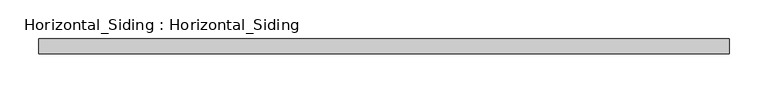
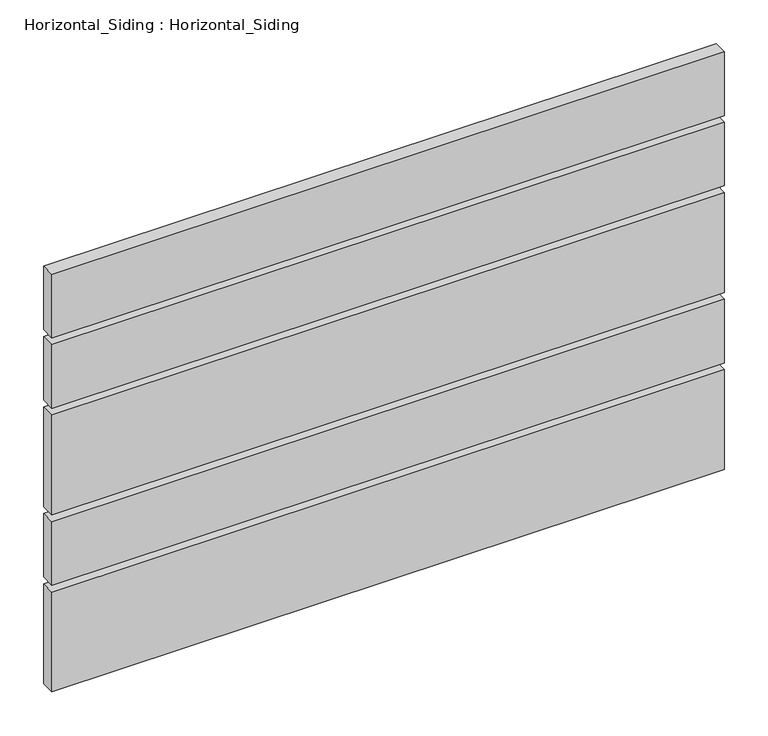
"""IFC4 building model written with IfcOpenShell, lengths in millimetres: plate geometry, Horizontal_Siding : Horizontal_Siding."""

from ifc_helpers import new_model, si_unit, frame, origin, place, context, project, spatial, polyline, outline, extrude, source, transform, mapped, element, save


def horizontal_siding_horizontal_siding_71e25863(model_context):
    return source(origin(), model_context, "Body", "SweptSolid", [
        extrude(outline(polyline([(444.5598994, -19.05), (-444.5598994, -19.05), (-444.5598994, 0.0), (444.5598994, 0.0), (444.5598994, -19.05)])), frame((0.0, 0.0, 9.525), z_axis=(0.0, 0.0, 1.0), x_axis=(1.0, 0.0, 0.0)), (0.0, 0.0, 1.0), 139.7),
        extrude(outline(polyline([(444.5598994, -19.05), (-444.5598994, -19.05), (-444.5598994, 0.0), (444.5598994, 0.0), (444.5598994, -19.05)])), frame((0.0, 0.0, 158.75), z_axis=(0.0, 0.0, 1.0), x_axis=(1.0, 0.0, 0.0)), (0.0, 0.0, 1.0), 88.9),
        extrude(outline(polyline([(444.5598994, -19.05), (-444.5598994, -19.05), (-444.5598994, 0.0), (444.5598994, 0.0), (444.5598994, -19.05)])), frame((0.0, 0.0, 257.175), z_axis=(0.0, 0.0, 1.0), x_axis=(1.0, 0.0, 0.0)), (0.0, 0.0, 1.0), 139.7),
        extrude(outline(polyline([(444.5598994, -19.05), (-444.5598994, -19.05), (-444.5598994, 0.0), (444.5598994, 0.0), (444.5598994, -19.05)])), frame((0.0, 0.0, 406.4), z_axis=(0.0, 0.0, 1.0), x_axis=(1.0, 0.0, 0.0)), (0.0, 0.0, 1.0), 88.9),
        extrude(outline(polyline([(444.5598994, -19.05), (-444.5598994, -19.05), (-444.5598994, 0.0), (444.5598994, 0.0), (444.5598994, -19.05)])), frame((0.0, 0.0, 504.825), z_axis=(0.0, 0.0, 1.0), x_axis=(1.0, 0.0, 0.0)), (0.0, 0.0, 1.0), 88.9),
    ])


if __name__ == "__main__":
    model = new_model("IFC4")
    model_context = context("Model", 3, world=origin())
    ifc_project = project(units=[si_unit("LENGTHUNIT", "METRE", prefix="MILLI")], contexts=[model_context])
    site = spatial("IfcSite", under=ifc_project)
    building = spatial("IfcBuilding", under=site)
    placement = place(None, origin())
    horizontal_siding_horizontal_siding_shape = horizontal_siding_horizontal_siding_71e25863(model_context)
    element("IfcPlate", 1, ObjectType="Horizontal_Siding : Horizontal_Siding", at=placement, inside=building, context=model_context, shape_type="MappedRepresentation", body=[
        mapped(horizontal_siding_horizontal_siding_shape, transform((0.0, 0.0, 0.0), x_axis=(1.0, 0.0, 0.0), y_axis=(0.0, 1.0, 0.0), z_axis=(0.0, 0.0, 1.0))),
    ])
    save(model, "model.ifc")

# Revit data of these elements
# Type "Horizontal_Siding : Horizontal_Siding"
#   Type Mark = "OUT"
#   Analytic Construction = "<None>"
#   extend = 0' - 2 3/4"
#   Width_2 = 0' - 3 1/2"
#   Width_1 = 0' - 5 1/2"
#   Gap = 0' - 0 3/8"
#   Plank Material = SLOTTED WOOD FENCE (THERMALLY MODIFIED WOOD: ARBOR WOOD)\n(EXTERIOR STAIN : PENOFIN VERDE EXT. STAIN - COLOR: CEDAR)
# Element 1 (IfcPlate, "Horizontal_Siding : Horizontal_Siding")
#   Materials on its faces: "SLOTTED WOOD FENCE (THERMALLY MODIFIED WOOD: ARBOR WOOD)\n(EXTERIOR STAIN : PENOFIN VERDE EXT. STAIN - COLOR: CEDAR)"
# Materials
#   "SLOTTED WOOD FENCE (THERMALLY MODIFIED WOOD: ARBOR WOOD)\n(EXTERIOR STAIN : PENOFIN VERDE EXT. STAIN - COLOR: CEDAR)": class "Wood", colour RGB 164 134 123, transparency 0, Description = "Pinus Echinata", Cost = 0
